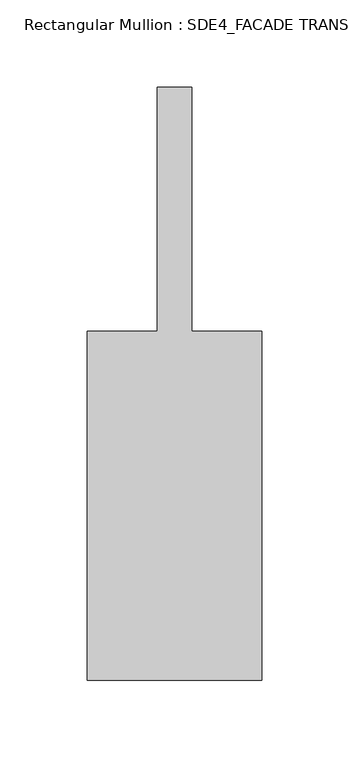
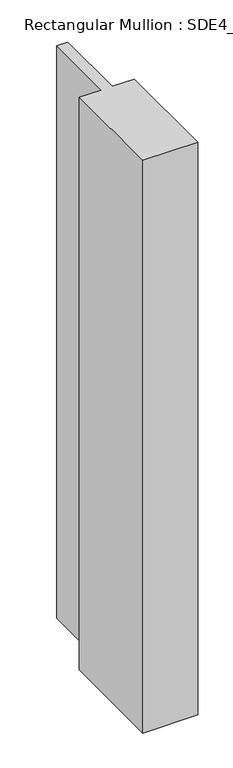
"""IFC4 building model written with IfcOpenShell, lengths in millimetres: member geometry, Rectangular Mullion : SDE4_FACADE TRANSOM TYPE 1."""

import ifcopenshell
import ifcopenshell.guid

model = None  # the IFC model being written
_history = None  # IfcOwnerHistory: only IFC2X3 demands one
_inside = {}  # id of a spatial element -> (the spatial element, [elements in it])
_under = {}  # id of a project, library or spatial element -> (it, [spatial elements below it])
_declared = {}  # id of a project -> (the project, [libraries it declares])
_typed = {}  # id of a type object -> (the type object, [elements of that type])
_made_of = {}  # id of a material, layer set ... -> (it, [elements and type objects made of it])


def new_model(schema):
    """Start an empty IFC model of exactly this schema.

    Asked for "IFC4X3", IfcOpenShell would pick the latest addendum, in which some entities
    have other attributes; the version numbers below select the first issue.
    IFC2X3 requires an IfcOwnerHistory on every rooted entity: one is made here for all.
    """
    global model, _history
    if schema == "IFC4X3":
        model = ifcopenshell.file(schema_version=(4, 3, 0, 0))
    else:
        model = ifcopenshell.file(schema=schema)
    _inside.clear()
    _under.clear()
    _declared.clear()
    _typed.clear()
    _made_of.clear()
    _history = None
    if model.schema == "IFC2X3":
        org = make("IfcOrganization", Name="unknown")
        user = make(
            "IfcPersonAndOrganization",
            ThePerson=make("IfcPerson", FamilyName="unknown"),
            TheOrganization=org,
        )
        app = make(
            "IfcApplication",
            ApplicationDeveloper=org,
            Version="unknown",
            ApplicationFullName="unknown",
            ApplicationIdentifier="unknown",
        )
        _history = make(
            "IfcOwnerHistory",
            OwningUser=user,
            OwningApplication=app,
            ChangeAction="ADDED",
            CreationDate=0,
        )
    return model


def make(cls, **values):
    """One entity of the class cls with the attributes given. An attribute that is None is left unset."""
    return model.create_entity(
        cls, **{name: value for name, value in values.items() if value is not None}
    )


def rooted(cls, **values):
    """An entity with a GlobalId (a new one), such as an element, a storey or a relation."""
    return make(cls, GlobalId=ifcopenshell.guid.new(), OwnerHistory=_history, **values)


def si_unit(unit_type, name, prefix=None):
    """IfcSIUnit, for example si_unit("LENGTHUNIT", "METRE", prefix="MILLI")."""
    return make("IfcSIUnit", UnitType=unit_type, Prefix=prefix, Name=name)


def assignment(units):
    """IfcUnitAssignment: the units of a project."""
    return None if units is None else make("IfcUnitAssignment", Units=units)


def point(xyz):
    """IfcCartesianPoint."""
    return None if xyz is None else make("IfcCartesianPoint", Coordinates=xyz)


def direction(xyz):
    """IfcDirection."""
    return None if xyz is None else make("IfcDirection", DirectionRatios=xyz)


def frame(location, z_axis=None, x_axis=None):
    """IfcAxis2Placement3D, a coordinate frame: its origin and axes. An axis left out is left unset."""
    return make(
        "IfcAxis2Placement3D",
        Location=point(location),
        Axis=direction(z_axis),
        RefDirection=direction(x_axis),
    )


def origin():
    """The frame at (0, 0, 0) with its axes left unset."""
    return frame((0.0, 0.0, 0.0))


def place(relative_to, where):
    """IfcLocalPlacement: puts the frame where relative to a parent placement (None: the world)."""
    return make(
        "IfcLocalPlacement", PlacementRelTo=relative_to, RelativePlacement=where
    )


def context(
    kind, dimensions, precision=None, world=None, true_north=None, identifier=None
):
    """IfcGeometricRepresentationContext, for example the 3D "Model" context."""
    return make(
        "IfcGeometricRepresentationContext",
        ContextIdentifier=identifier,
        ContextType=kind,
        CoordinateSpaceDimension=dimensions,
        Precision=precision,
        WorldCoordinateSystem=world,
        TrueNorth=true_north,
    )


def project(units=None, contexts=None):
    """IfcProject with its units and contexts."""
    return rooted(
        "IfcProject",
        Name="project",
        RepresentationContexts=contexts,
        UnitsInContext=assignment(units),
    )


def spatial(cls, under=None, at=None, **own):
    """A site, building, storey or space (cls), placed at a placement, below another one or the project."""
    s = rooted(cls, ObjectPlacement=at, **own)
    if under is not None:
        _under.setdefault(under.id(), (under, []))[1].append(s)
    return s


def polyline(points):
    """IfcPolyline through the points."""
    return make("IfcPolyline", Points=[point(p) for p in points])


def outline(outer, holes=None, kind="AREA"):
    """IfcArbitraryClosedProfileDef: a profile drawn as a closed curve; with holes, ...WithVoids."""
    if holes is None:
        return make("IfcArbitraryClosedProfileDef", ProfileType=kind, OuterCurve=outer)
    return make(
        "IfcArbitraryProfileDefWithVoids",
        ProfileType=kind,
        OuterCurve=outer,
        InnerCurves=holes,
    )


def extrude(swept, where, along, depth):
    """IfcExtrudedAreaSolid: the profile swept, set in the frame where, extruded along a direction by depth."""
    return make(
        "IfcExtrudedAreaSolid",
        SweptArea=swept,
        Position=where,
        ExtrudedDirection=direction(along),
        Depth=depth,
    )


def shape(context_of_items, identifier, shape_type, items):
    """IfcShapeRepresentation: the items that make up one representation, for example the "Body"."""
    return make(
        "IfcShapeRepresentation",
        ContextOfItems=context_of_items,
        RepresentationIdentifier=identifier,
        RepresentationType=shape_type,
        Items=items,
    )


def source(mapping_origin, context_of_items, identifier, shape_type, items):
    """IfcRepresentationMap: a shape defined once, which mapped items show again and again."""
    return make(
        "IfcRepresentationMap",
        MappingOrigin=mapping_origin,
        MappedRepresentation=shape(context_of_items, identifier, shape_type, items),
    )


def transform(
    local_origin,
    x_axis=None,
    y_axis=None,
    z_axis=None,
    scale=None,
    scale2=None,
    scale3=None,
    uniform=True,
):
    """IfcCartesianTransformationOperator3D, or its non-uniform kind. x_axis, y_axis, z_axis: its Axis1, 2, 3."""
    if uniform:
        return make(
            "IfcCartesianTransformationOperator3D",
            Axis1=direction(x_axis),
            Axis2=direction(y_axis),
            LocalOrigin=point(local_origin),
            Scale=scale,
            Axis3=direction(z_axis),
        )
    return make(
        "IfcCartesianTransformationOperator3DnonUniform",
        Axis1=direction(x_axis),
        Axis2=direction(y_axis),
        LocalOrigin=point(local_origin),
        Scale=scale,
        Axis3=direction(z_axis),
        Scale2=scale2,
        Scale3=scale3,
    )


def mapped(mapping_source, mapping_target):
    """IfcMappedItem: shows the shape of a source again, moved by a transform."""
    return make(
        "IfcMappedItem", MappingSource=mapping_source, MappingTarget=mapping_target
    )


def made_of(thing, what):
    """Note that an element or type object is made of a material, layer set ...; save() writes the relation."""
    if what is not None:
        _made_of.setdefault(what.id(), (what, []))[1].append(thing)
    return thing


def element(
    cls,
    number,
    at=None,
    inside=None,
    cuts=None,
    type_object=None,
    material=None,
    context=None,
    identifier="Body",
    shape_type=None,
    held_by="IfcProductDefinitionShape",
    body=None,
    shapes=None,
    **own,
):
    """One element of the class cls, such as IfcWall. Its Tag is "e" and its number.

    at: its placement. inside: the storey or other place that contains it. cuts: it is an
    opening in that element (IfcRelVoidsElement). A single representation is given by context,
    identifier, shape_type and body (its items); several are given by shapes. held_by: the class
    of the entity that holds the representations. save() writes the other relations.
    """
    e = rooted(cls, Tag="e%d" % number, ObjectPlacement=at, **own)
    if body is not None:
        shapes = [shape(context, identifier, shape_type, body)]
    if shapes is not None:
        e.Representation = make(held_by, Representations=shapes)
    if inside is not None:
        _inside.setdefault(inside.id(), (inside, []))[1].append(e)
    if cuts is not None:
        rooted(
            "IfcRelVoidsElement", RelatingBuildingElement=cuts, RelatedOpeningElement=e
        )
    if type_object is not None:
        _typed.setdefault(type_object.id(), (type_object, []))[1].append(e)
    return made_of(e, material)


def aggregate(whole, parts):
    """IfcRelAggregates: a whole, such as a stair, and the parts it consists of."""
    return rooted("IfcRelAggregates", RelatingObject=whole, RelatedObjects=parts)


def save(model, path):
    """Write the relations noted so far, then the file.

    IfcRelAggregates (storeys below a building ...), IfcRelContainedInSpatialStructure (elements
    in a storey), IfcRelDefinesByType, IfcRelAssociatesMaterial and IfcRelDeclares: one each for
    every whole, place, type object, material and project.
    """
    for whole, parts in _under.values():
        aggregate(whole, parts)
    for where, things in _inside.values():
        rooted(
            "IfcRelContainedInSpatialStructure",
            RelatedElements=things,
            RelatingStructure=where,
        )
    for kind, things in _typed.values():
        rooted("IfcRelDefinesByType", RelatedObjects=things, RelatingType=kind)
    for what, things in _made_of.values():
        rooted("IfcRelAssociatesMaterial", RelatedObjects=things, RelatingMaterial=what)
    for by, libraries in _declared.values():
        rooted("IfcRelDeclares", RelatingContext=by, RelatedDefinitions=libraries)
    model.write(path)


def rectangular_mullion_sde4_facade_transom_type_1_2e3f63cd(model_context):
    return source(origin(), model_context, "Body", "SweptSolid", [
        extrude(outline(polyline([(50.0, -132.5), (-50.0, -132.5), (-50.0, 67.5), (-10.0, 67.5), (-10.0, 207.5), (10.0, 207.5), (10.0, 67.5), (50.0, 67.5), (50.0, -132.5)])), frame((0.0, 0.0, -1100.0), z_axis=(0.0, 0.0, 1.0), x_axis=(1.0, 0.0, 0.0)), (0.0, 0.0, 1.0), 1100.0),
    ])


if __name__ == "__main__":
    model = new_model("IFC4")
    model_context = context("Model", 3, world=origin())
    ifc_project = project(units=[si_unit("LENGTHUNIT", "METRE", prefix="MILLI")], contexts=[model_context])
    site = spatial("IfcSite", under=ifc_project)
    building = spatial("IfcBuilding", under=site)
    placement = place(None, origin())
    rectangular_mullion_sde4_facade_transom_type_1_shape = rectangular_mullion_sde4_facade_transom_type_1_2e3f63cd(model_context)
    element("IfcMember", 1, ObjectType="Rectangular Mullion : SDE4_FACADE TRANSOM TYPE 1", at=placement, inside=building, context=model_context, shape_type="MappedRepresentation", body=[
        mapped(rectangular_mullion_sde4_facade_transom_type_1_shape, transform((0.0, 0.0, 0.0), x_axis=(1.0, 0.0, 0.0), y_axis=(0.0, 1.0, 0.0), z_axis=(0.0, 0.0, 1.0))),
    ])
    save(model, "model.ifc")

# Revit data of these elements
# Type "Rectangular Mullion : SDE4_FACADE TRANSOM TYPE 1"
#   built-in parameter 1007322 = 1.11549 (stored number, unit not read)
#   built-in parameter 1007321 = 0.164042 (stored number, unit not read)
#   built-in parameter 1007320 = 0.164042 (stored number, unit not read)
